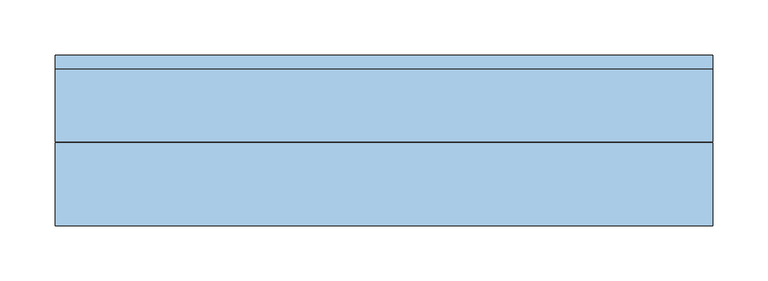
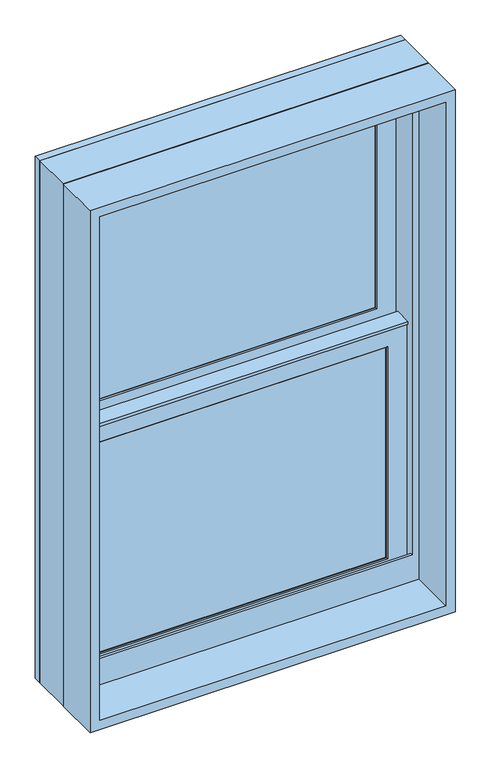
"""IFC4 building model written with IfcOpenShell, lengths in millimetres: window geometry, Window-Double_Hung-Marvin-Essential : ESDH2030."""

from ifc_helpers import new_model, si_unit, frame, origin, place, context, project, spatial, polyline, outline, extrude, faceted_brep, source, transform, mapped, element, save


def window_959f815f(model_context):
    return source(origin(), model_context, "Body", "SolidModel", [
        extrude(outline(polyline([(89.9583333, 20.6375), (89.9583333, 15.875), (70.9083333, 15.875), (70.9083333, 20.6375), (89.9583333, 20.6375)])), frame((0.0, 0.0, 1593.85), z_axis=(0.0, 0.0, 1.0), x_axis=(1.0, 0.0, 0.0)), (0.0, 0.0, 1.0), 374.65),
        extrude(outline(polyline([(-70.9083333, 20.6375), (-70.9083333, 15.875), (-89.9583333, 15.875), (-89.9583333, 20.6375), (-70.9083333, 20.6375)])), frame((0.0, 0.0, 1593.85), z_axis=(0.0, 0.0, 1.0), x_axis=(1.0, 0.0, 0.0)), (0.0, 0.0, 1.0), 374.65),
        extrude(outline(polyline([(241.3, 20.6375), (241.3, 15.875), (-241.3, 15.875), (-241.3, 20.6375), (241.3, 20.6375)])), frame((0.0, 0.0, 1771.65), z_axis=(0.0, 0.0, 1.0), x_axis=(1.0, 0.0, 0.0)), (0.0, 0.0, 1.0), 19.05),
        extrude(outline(polyline([(-89.9583333, 46.83125), (-89.9583333, 51.59375), (-70.9083333, 51.59375), (-70.9083333, 46.83125), (-89.9583333, 46.83125)])), frame((0.0, 0.0, 2006.6), z_axis=(0.0, 0.0, 1.0), x_axis=(1.0, 0.0, 0.0)), (0.0, 0.0, 1.0), 374.65),
        extrude(outline(polyline([(70.9083333, 46.83125), (70.9083333, 51.59375), (89.9583333, 51.59375), (89.9583333, 46.83125), (70.9083333, 46.83125)])), frame((0.0, 0.0, 2006.6), z_axis=(0.0, 0.0, 1.0), x_axis=(1.0, 0.0, 0.0)), (0.0, 0.0, 1.0), 374.65),
        extrude(outline(polyline([(-241.3, 46.83125), (-241.3, 51.59375), (241.3, 51.59375), (241.3, 46.83125), (-241.3, 46.83125)])), frame((0.0, 0.0, 2184.4), z_axis=(0.0, 0.0, 1.0), x_axis=(1.0, 0.0, 0.0)), (0.0, 0.0, 1.0), 19.05),
        extrude(outline(polyline([(89.9583333, 20.6375), (70.9083333, 20.6375), (70.9083333, 25.4), (89.9583333, 25.4), (89.9583333, 20.6375)])), frame((0.0, 0.0, 1593.85), z_axis=(0.0, 0.0, 1.0), x_axis=(1.0, 0.0, 0.0)), (0.0, 0.0, 1.0), 374.65),
        extrude(outline(polyline([(-70.9083333, 20.6375), (-89.9583333, 20.6375), (-89.9583333, 25.4), (-70.9083333, 25.4), (-70.9083333, 20.6375)])), frame((0.0, 0.0, 1593.85), z_axis=(0.0, 0.0, 1.0), x_axis=(1.0, 0.0, 0.0)), (0.0, 0.0, 1.0), 374.65),
        extrude(outline(polyline([(241.3, 20.6375), (-241.3, 20.6375), (-241.3, 25.4), (241.3, 25.4), (241.3, 20.6375)])), frame((0.0, 0.0, 1771.65), z_axis=(0.0, 0.0, 1.0), x_axis=(1.0, 0.0, 0.0)), (0.0, 0.0, 1.0), 19.05),
        extrude(outline(polyline([(-89.9583333, 56.35625), (-70.9083333, 56.35625), (-70.9083333, 51.59375), (-89.9583333, 51.59375), (-89.9583333, 56.35625)])), frame((0.0, 0.0, 2006.6), z_axis=(0.0, 0.0, 1.0), x_axis=(1.0, 0.0, 0.0)), (0.0, 0.0, 1.0), 374.65),
        extrude(outline(polyline([(70.9083333, 56.35625), (89.9583333, 56.35625), (89.9583333, 51.59375), (70.9083333, 51.59375), (70.9083333, 56.35625)])), frame((0.0, 0.0, 2006.6), z_axis=(0.0, 0.0, 1.0), x_axis=(1.0, 0.0, 0.0)), (0.0, 0.0, 1.0), 374.65),
        extrude(outline(polyline([(-241.3, 56.35625), (241.3, 56.35625), (241.3, 51.59375), (-241.3, 51.59375), (-241.3, 56.35625)])), frame((0.0, 0.0, 2184.4), z_axis=(0.0, 0.0, 1.0), x_axis=(1.0, 0.0, 0.0)), (0.0, 0.0, 1.0), 19.05),
        faceted_brep([(-268.2875, 5.6780605, 1998.5351748), (-268.2875, 5.6780605, 1993.9), (268.2875, 5.6780605, 1993.9), (268.2875, 5.6780605, 1998.5351748), (-268.2875, 34.8118605, 1998.5351748), (268.2875, 34.8118605, 1998.5351748), (268.2875, 34.8118605, 1993.9), (-268.2875, 34.8118605, 1993.9), (-268.2875, 30.1625, 1993.9), (-268.2875, 30.1625, 1566.8625), (-268.2875, 8.9241104, 1566.8625), (-268.2875, 8.9241104, 1993.9), (268.2875, 8.9241104, 1993.9), (268.2875, 30.1625, 1993.9), (268.2875, 8.9241104, 1566.8625), (268.2875, 30.1625, 1566.8625), (-252.4034752, 11.90625, 1979.6034752), (-252.4034752, 30.1625, 1979.6034752), (252.4034752, 30.1625, 1979.6034752), (252.4034752, 11.90625, 1979.6034752), (-235.74375, 10.4662439, 1962.94375), (-235.74375, 11.90625, 1962.94375), (235.74375, 11.90625, 1962.94375), (235.74375, 10.4662439, 1962.94375), (237.2858834, 8.9241104, 1964.4858834), (-237.2858834, 8.9241104, 1964.4858834), (252.4034752, 30.1625, 1582.7465248), (252.4034752, 11.90625, 1582.7465248), (235.74375, 11.90625, 1599.40625), (235.74375, 10.4662439, 1599.40625), (237.2858834, 8.9241104, 1597.8641166), (-252.4034752, 30.1625, 1582.7465248), (-252.4034752, 11.90625, 1582.7465248), (-235.74375, 11.90625, 1599.40625), (-235.74375, 10.4662439, 1599.40625), (-237.2858834, 8.9241104, 1597.8641166)], [[[0, 1, 2, 3]], [[4, 5, 6, 7]], [[1, 0, 4, 7, 8, 9, 10, 11]], [[2, 1, 11, 12]], [[7, 6, 13, 8]], [[3, 2, 12, 14, 15, 13, 6, 5]], [[0, 3, 5, 4]], [[16, 17, 18, 19]], [[20, 21, 22, 23]], [[20, 23, 24, 25]], [[19, 18, 26, 27]], [[23, 22, 28, 29]], [[24, 23, 29, 30]], [[27, 26, 31, 32]], [[29, 28, 33, 34]], [[30, 29, 34, 35]], [[15, 14, 10, 9]], [[15, 9, 8, 13], [18, 17, 31, 26]], [[17, 16, 32, 31]], [[16, 19, 27, 32], [22, 21, 33, 28]], [[21, 20, 34, 33]], [[20, 25, 35, 34]], [[10, 14, 12, 11], [25, 24, 30, 35]]]),
        extrude(outline(polyline([(38.5955581, 1979.6125), (33.5778968, 1979.6125), (33.5778968, 1981.2), (39.9405976, 1981.2), (39.9405976, 1979.6125), (61.515625, 1979.6125), (47.6307501, 1976.2975159), (38.5955581, 1976.2975159), (38.5955581, 1979.6125)])), frame((-268.2875, 0.0, 0.0), z_axis=(1.0, 0.0, 0.0), x_axis=(0.0, 1.0, 0.0)), (0.0, 0.0, 1.0), 536.575),
        faceted_brep([(298.45, 0.0, 1536.7), (298.45, 0.0, 2438.4), (-298.45, 0.0, 2438.4), (-298.45, 0.0, 1536.7), (272.25625, 0.0, 1597.81875), (-272.25625, 0.0, 1597.81875), (-272.25625, 0.0, 2412.20625), (272.25625, 0.0, 2412.20625), (272.25625, 3.96875, 1536.7), (-272.25625, 3.96875, 1536.7), (-272.25625, 3.96875, 1597.81875), (272.25625, 3.96875, 1597.81875), (-298.45, 65.6828125, 1536.7), (-272.25625, 65.6828125, 1536.7), (272.25625, 65.6828125, 1536.7), (298.45, 65.6828125, 1536.7), (-298.45, 65.6828125, 2438.4), (298.45, 65.6828125, 2438.4), (272.25625, 65.6828125, 2412.20625), (-272.25625, 65.6828125, 2412.20625)], [[[0, 1, 2, 3], [4, 5, 6, 7]], [[8, 9, 10, 11]], [[5, 4, 11, 10]], [[0, 3, 12, 13, 9, 8, 14, 15]], [[13, 12, 16, 17, 15, 14, 18, 19]], [[13, 19, 6, 5, 10, 9]], [[7, 6, 19, 18]], [[18, 14, 8, 11, 4, 7]], [[1, 0, 15, 17]], [[2, 1, 17, 16]], [[3, 2, 16, 12]]]),
        faceted_brep([(272.25625, 30.1625, 1987.55), (270.66875, 30.1625, 1987.55), (270.66875, 30.1625, 1561.0544613), (272.25625, 30.1625, 1561.0544613), (-270.66875, 30.1625, 1987.55), (-272.25625, 30.1625, 1987.55), (-272.25625, 30.1625, 1561.0544613), (-270.66875, 30.1625, 1561.0544613), (270.66875, 63.5, 1987.55), (272.25625, 63.5, 1987.55), (272.25625, 63.5, 1554.5743077), (270.66875, 63.5, 1554.5743077), (-272.25625, 63.5, 1987.55), (-270.66875, 63.5, 1987.55), (-270.66875, 63.5, 1554.5743077), (-272.25625, 63.5, 1554.5743077), (283.5108932, 3.96875, 1566.1460105), (283.5108932, 3.96875, 1536.7), (283.5108932, 65.6828125, 1536.7), (283.5108932, 65.6828125, 1554.150012), (-283.5108932, 3.96875, 1536.7), (-283.5108932, 3.96875, 1566.1460105), (-283.5108932, 65.6828125, 1554.150012), (-283.5108932, 65.6828125, 1536.7), (283.5108932, 78.58125, 1551.6428097), (-283.5108932, 78.58125, 1551.6428097), (-281.4971252, 68.2348864, 1553.6539391), (-263.53135, 68.2348864, 1553.6539391), (-263.53135, 65.6828125, 1554.150012), (263.53135, 65.6828125, 1554.150012), (263.53135, 68.2348864, 1553.6539391), (281.4971252, 68.2348864, 1553.6539391), (-298.45, 65.6828125, 1536.7), (-298.45, 78.5948249, 1536.7), (298.45, 78.5948249, 1536.7), (298.45, 65.6828125, 1536.7), (-298.45, 78.58125, 2438.4), (298.45, 78.58125, 2438.4), (283.5108932, 78.58125, 2423.4608932), (-283.5108932, 78.58125, 2423.4608932), (-298.45, 65.6828125, 2438.4), (-281.4971252, 68.2348864, 2421.4471252), (281.4971252, 68.2348864, 2421.4471252), (263.53135, 68.2348864, 2403.48135), (-263.53135, 68.2348864, 2403.48135), (-263.53135, 65.6828125, 2403.48135), (263.53135, 65.6828125, 2403.48135), (298.45, 65.6828125, 2438.4)], [[[0, 1, 2, 3]], [[4, 5, 6, 7]], [[8, 9, 10, 11]], [[12, 13, 14, 15]], [[1, 8, 11, 2]], [[9, 0, 3, 10]], [[1, 0, 9, 8]], [[5, 4, 13, 12]], [[5, 12, 15, 6]], [[13, 4, 7, 14]], [[16, 17, 18, 19]], [[20, 21, 22, 23]], [[24, 25, 26, 27, 28, 22, 21, 16, 19, 29, 30, 31], [3, 2, 11, 10], [7, 6, 15, 14]], [[17, 16, 21, 20]], [[17, 20, 23, 32, 33, 34, 35, 18]], [[34, 33, 36, 37], [25, 24, 38, 39]], [[33, 32, 40, 36]], [[39, 41, 26, 25]], [[41, 42, 31, 30, 43, 44, 27, 26]], [[44, 45, 28, 27]], [[40, 32, 23, 22, 28, 45, 46, 29, 19, 18, 35, 47]], [[36, 40, 47, 37]], [[39, 38, 42, 41]], [[44, 43, 46, 45]], [[34, 37, 47, 35]], [[42, 38, 24, 31]], [[46, 43, 30, 29]]]),
        extrude(outline(polyline([(248.44375, 11.90625), (-248.44375, 11.90625), (-248.44375, 15.08125), (248.44375, 15.08125), (248.44375, 11.90625)])), frame((0.0, 0.0, 1586.70625), z_axis=(0.0, 0.0, 1.0), x_axis=(1.0, 0.0, 0.0)), (0.0, 0.0, 1.0), 388.9375),
        extrude(outline(polyline([(248.44375, 42.8625), (-248.44375, 42.8625), (-248.44375, 46.0375), (248.44375, 46.0375), (248.44375, 42.8625)])), frame((0.0, 0.0, 1999.45625), z_axis=(0.0, 0.0, 1.0), x_axis=(1.0, 0.0, 0.0)), (0.0, 0.0, 1.0), 388.9375),
        faceted_brep([(-235.74375, 31.194477, 1962.94375), (-237.2858834, 32.7366104, 1964.4858834), (237.2858834, 32.7366104, 1964.4858834), (235.74375, 31.194477, 1962.94375), (-235.74375, 30.1625, 1962.94375), (235.74375, 30.1625, 1962.94375), (-268.2875, 32.7366104, 1995.4875), (-268.2875, 30.1625, 1995.4875), (268.2875, 30.1625, 1995.4875), (268.2875, 32.7366104, 1995.4875), (237.2858834, 32.7366104, 1597.8641166), (235.74375, 31.194477, 1599.40625), (235.74375, 30.1625, 1599.40625), (268.2875, 30.1625, 1566.8625), (268.2875, 32.7366104, 1566.8625), (-237.2858834, 32.7366104, 1597.8641166), (-235.74375, 31.194477, 1599.40625), (-235.74375, 30.1625, 1599.40625), (-268.2875, 30.1625, 1566.8625), (-268.2875, 32.7366104, 1566.8625)], [[[0, 1, 2, 3]], [[4, 0, 3, 5]], [[6, 7, 8, 9]], [[3, 2, 10, 11]], [[5, 3, 11, 12]], [[9, 8, 13, 14]], [[11, 10, 15, 16]], [[12, 11, 16, 17]], [[14, 13, 18, 19]], [[9, 14, 19, 6], [1, 15, 10, 2]], [[16, 15, 1, 0]], [[17, 16, 0, 4]], [[7, 18, 13, 8], [5, 12, 17, 4]], [[19, 18, 7, 6]]]),
        faceted_brep([(-252.4034752, 42.8625, 2392.3534752), (-252.4034752, 61.11875, 2392.3534752), (252.4034752, 61.11875, 2392.3534752), (252.4034752, 42.8625, 2392.3534752), (-235.74375, 41.4224939, 2375.69375), (-235.74375, 42.8625, 2375.69375), (235.74375, 42.8625, 2375.69375), (235.74375, 41.4224939, 2375.69375), (-237.2858834, 39.8803604, 2377.2358834), (237.2858834, 39.8803604, 2377.2358834), (-268.2875, 61.11875, 2408.2375), (-268.2875, 39.8803604, 2408.2375), (268.2875, 39.8803604, 2408.2375), (268.2875, 61.11875, 2408.2375), (252.4034752, 61.11875, 1995.4965248), (252.4034752, 42.8625, 1995.4965248), (235.74375, 42.8625, 2012.15625), (235.74375, 41.4224939, 2012.15625), (237.2858834, 39.8803604, 2010.6141166), (268.2875, 39.8803604, 1979.6125), (268.2875, 61.11875, 1979.6125), (-252.4034752, 61.11875, 1995.4965248), (-252.4034752, 42.8625, 1995.4965248), (-235.74375, 42.8625, 2012.15625), (-235.74375, 41.4224939, 2012.15625), (-237.2858834, 39.8803604, 2010.6141166), (-268.2875, 39.8803604, 1979.6125), (-268.2875, 61.11875, 1979.6125)], [[[0, 1, 2, 3]], [[4, 5, 6, 7]], [[8, 4, 7, 9]], [[10, 11, 12, 13]], [[3, 2, 14, 15]], [[7, 6, 16, 17]], [[9, 7, 17, 18]], [[13, 12, 19, 20]], [[15, 14, 21, 22]], [[17, 16, 23, 24]], [[18, 17, 24, 25]], [[20, 19, 26, 27]], [[13, 20, 27, 10], [1, 21, 14, 2]], [[22, 21, 1, 0]], [[3, 15, 22, 0], [5, 23, 16, 6]], [[24, 23, 5, 4]], [[25, 24, 4, 8]], [[11, 26, 19, 12], [9, 18, 25, 8]], [[27, 26, 11, 10]]]),
        faceted_brep([(-268.2875, 61.11875, 1979.6125), (-268.2875, 63.6928604, 1979.6125), (268.2875, 63.6928604, 1979.6125), (268.2875, 61.11875, 1979.6125), (-235.74375, 62.150727, 2012.15625), (-235.74375, 61.11875, 2012.15625), (235.74375, 61.11875, 2012.15625), (235.74375, 62.150727, 2012.15625), (-237.2858834, 63.6928604, 2010.6141166), (237.2858834, 63.6928604, 2010.6141166), (268.2875, 63.6928604, 2408.2375), (268.2875, 61.11875, 2408.2375), (235.74375, 61.11875, 2375.69375), (235.74375, 62.150727, 2375.69375), (237.2858834, 63.6928604, 2377.2358834), (-268.2875, 63.6928604, 2408.2375), (-268.2875, 61.11875, 2408.2375), (-235.74375, 61.11875, 2375.69375), (-235.74375, 62.150727, 2375.69375), (-237.2858834, 63.6928604, 2377.2358834)], [[[0, 1, 2, 3]], [[4, 5, 6, 7]], [[8, 4, 7, 9]], [[3, 2, 10, 11]], [[7, 6, 12, 13]], [[9, 7, 13, 14]], [[11, 10, 15, 16]], [[13, 12, 17, 18]], [[14, 13, 18, 19]], [[16, 15, 1, 0]], [[3, 11, 16, 0], [5, 17, 12, 6]], [[18, 17, 5, 4]], [[19, 18, 4, 8]], [[1, 15, 10, 2], [9, 14, 19, 8]]]),
        extrude(outline(polyline([(248.44375, 26.19375), (-248.44375, 26.19375), (-248.44375, 30.1625), (248.44375, 30.1625), (248.44375, 26.19375)])), frame((0.0, 0.0, 1586.70625), z_axis=(0.0, 0.0, 1.0), x_axis=(1.0, 0.0, 0.0)), (0.0, 0.0, 1.0), 388.9375),
        extrude(outline(polyline([(248.44375, 57.15), (-248.44375, 57.15), (-248.44375, 61.11875), (248.44375, 61.11875), (248.44375, 57.15)])), frame((0.0, 0.0, 1999.45625), z_axis=(0.0, 0.0, 1.0), x_axis=(1.0, 0.0, 0.0)), (0.0, 0.0, 1.0), 388.9375),
        extrude(outline(polyline([(2438.4, 298.45), (2438.4, -298.45), (1536.7, -298.45), (1536.7, 298.45), (2438.4, 298.45)]), holes=[polyline([(2422.525, 282.575), (1552.575, 282.575), (1552.575, -282.575), (2422.525, -282.575), (2422.525, 282.575)])]), frame((0.0, -76.2, 0.0), z_axis=(0.0, 1.0, 0.0), x_axis=(0.0, 0.0, 1.0)), (0.0, 0.0, 1.0), 75.40625),
    ])


if __name__ == "__main__":
    model = new_model("IFC4")
    model_context = context("Model", 3, world=origin())
    ifc_project = project(units=[si_unit("LENGTHUNIT", "METRE", prefix="MILLI")], contexts=[model_context])
    site = spatial("IfcSite", under=ifc_project)
    building = spatial("IfcBuilding", under=site)
    placement = place(None, origin())
    window_shape = window_959f815f(model_context)
    element("IfcWindow", 1, ObjectType="Window-Double_Hung-Marvin-Essential : ESDH2030", at=placement, inside=building, context=model_context, shape_type="MappedRepresentation", body=[
        mapped(window_shape, transform((0.0, 0.0, 0.0), x_axis=(1.0, 0.0, 0.0), y_axis=(0.0, 1.0, 0.0), z_axis=(0.0, 0.0, 1.0))),
    ])
    save(model, "model.ifc")

# Revit data of these elements
# Type "Window-Double_Hung-Marvin-Essential : ESDH2030"
#   Type Mark = "34"
#   Window Type = "Essential Double Hung"
#   Product data url = "https://bimobject.com/marvin-windows-and-doors/product/marvin-dhwau"
#   Product Guid = "c4a96547-874c-4385-91dc-a058adc19d98"
#   Frame = "All Ultrex"
#   Egress Window = "No"
#   URL = "www.marvin.com"
#   Model = "ESDH2030"
#   Manufacturer = "Marvin Windows and Doors"
#   Label Egress = ""
#   Glass Type = "IG Low E II with Argon"
#   Design Pressure = "DP50"
#   Description = "2436 DBHG"
#   Analytic Construction = "<None>"
#   Prairie Corner Width = 0' - 4"
#   Prairie Corner Height = 0' - 4"
#   Egress Width = 1' - 8 9/16"
#   Egress Height = 1' - 1 27/128"
#   Rough Width = 2' - 0"
#   Rough Height = 3' - 0"
#   Nominal Width = 2' - 0"
#   Nominal Height = 3' - 0"
#   Inset to Installation Flange [instance default] = 0' - 1"
#   Height = 2' - 11 1/2"
#   Egress Area = 1.88646 SF
#   Default Head Height = 8' - 0"
#   Width = 1' - 11 1/2"
#   Daylight Area = 3.68994 SF
#   DLO Width = 1' - 6 9/16"
#   DLO Height = 1' - 2 5/16"
#   Muntins Top Sash = yes
#   Lites Wide Top Sash = 3
#   Lites Wide Bottom Sash = 3
#   Lites High Top Sash = 2
#   Lites High Bottom Sash = 2
#   Lite Cut Prairie 9 = no
#   Lite Cut HV Grid = yes
#   Muntins Bottom Sash = yes
#   Label Visibility = no
#   Jamb Extension Visibility = yes
#   Edition number = 1
#   Interior Material = Ultrex-Marvin-Stonewhite
#   Glazing Material = Glass-Marvin-IG Low E II with Argon
#   Cladding Material = Ultrex-Marvin-Pebblegray
#   Wall Closure = (empty or 0)
#   Assembly Code = ""
# Element 1 (IfcWindow, "Window-Double_Hung-Marvin-Essential : ESDH2030")
#   Materials on its faces: "Ultrex-Marvin-Pebblegray", "Ultrex-Marvin-Stonewhite", "Glass-Marvin-IG Low E II with Argon"
# Materials
#   "Ultrex-Marvin-Stonewhite": class "Paint", colour RGB 250 251 245, transparency 0
#   "Glass-Marvin-IG Low E II with Argon": class "Glass", colour RGB 0 128 192, transparency 0.85
#   "Ultrex-Marvin-Pebblegray": class "Paint", colour RGB 189 185 173, transparency 0
